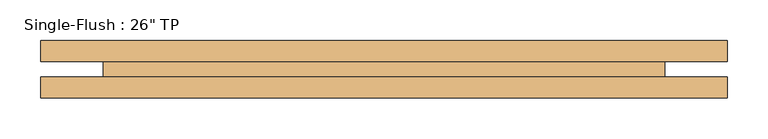
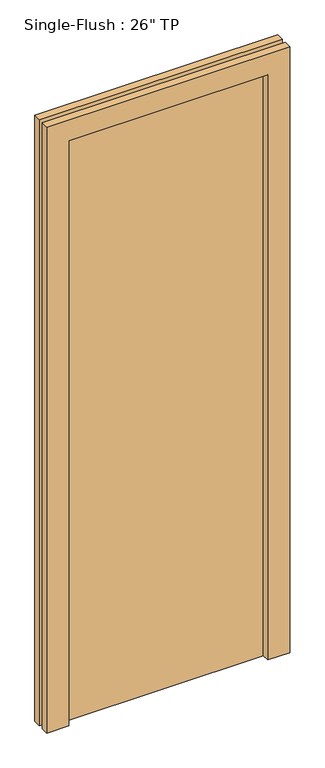
"""IFC4 building model written with IfcOpenShell, lengths in millimetres: door geometry."""

from ifc_helpers import new_model, si_unit, frame, origin, origin_with_axes, place, context, project, spatial, polyline, outline, extrude, source, transform, mapped, element, save


def door_5b9545ad(model_context):
    return source(origin(), model_context, "Body", "SweptSolid", [
        extrude(outline(polyline([(2209.8, -419.1), (0.0, -419.1), (0.0, -342.9), (2133.6, -342.9), (2133.6, 342.9), (0.0, 342.9), (0.0, 419.1), (2209.8, 419.1), (2209.8, -419.1)])), frame((0.0, 9.525, 0.0), z_axis=(0.0, 1.0, 0.0), x_axis=(0.0, 0.0, 1.0)), (0.0, 0.0, 1.0), 25.4),
        extrude(outline(polyline([(2209.8, 419.1), (2209.8, -419.1), (0.0, -419.1), (0.0, -342.9), (2133.6, -342.9), (2133.6, 342.9), (0.0, 342.9), (0.0, 419.1), (2209.8, 419.1)])), frame((0.0, -34.925, 0.0), z_axis=(0.0, 1.0, 0.0), x_axis=(0.0, 0.0, 1.0)), (0.0, 0.0, 1.0), 25.4),
        extrude(outline(polyline([(342.9, -9.525), (-342.9, -9.525), (-342.9, 9.525), (342.9, 9.525), (342.9, -9.525)])), origin_with_axes(), (0.0, 0.0, 1.0), 2133.6),
    ])


if __name__ == "__main__":
    model = new_model("IFC4")
    model_context = context("Model", 3, world=origin())
    ifc_project = project(units=[si_unit("LENGTHUNIT", "METRE", prefix="MILLI")], contexts=[model_context])
    site = spatial("IfcSite", under=ifc_project)
    building = spatial("IfcBuilding", under=site)
    placement = place(None, origin())
    door_shape = door_5b9545ad(model_context)
    element("IfcDoor", 1, ObjectType="Single-Flush : 26\" TP", at=placement, inside=building, context=model_context, shape_type="MappedRepresentation", body=[
        mapped(door_shape, transform((0.0, 0.0, 0.0), x_axis=(1.0, 0.0, 0.0), y_axis=(0.0, 1.0, 0.0), z_axis=(0.0, 0.0, 1.0))),
    ])
    save(model, "model.ifc")

# Revit data of these elements
# Type "Single-Flush : 26\" TP"
#   Type Mark = "56"
#   Construction Type Id = "MDOOR"
#   Assembly Code = "C1020"
#   Analytic Construction = "Metal"
#   Thickness = 0' - 0 3/4"
#   Heat Transfer Coefficient (U) = 3.7021 W/(m²·K)
#   Height = 7' - 0"
#   Trim Projection Ext = 0' - 1"
#   Trim Projection Int = 0' - 1"
#   Trim Width = 0' - 3"
#   Width = 2' - 3"
#   Door Material = Door - Panel
#   Frame Material = Door - Frame
#   Visual Light Transmittance = 0
#   Solar Heat Gain Coefficient = 0
#   Function = (empty or 0)
#   Wall Closure = (empty or 0)
# Element 1 (IfcDoor, "Single-Flush : 26\" TP")
#   Materials on its faces: "Door - Frame", "Door - Panel"
# Materials
#   "Door - Panel": class "Wood", colour RGB 210 159 95, transparency 0
#   "Door - Frame": class "Miscellaneous", colour RGB 118 70 51, transparency 0
